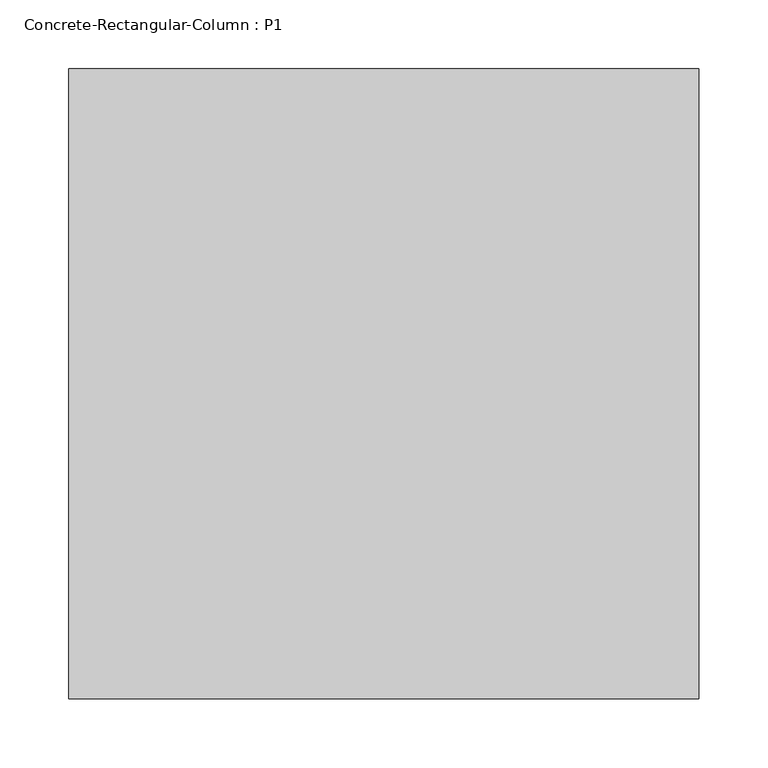
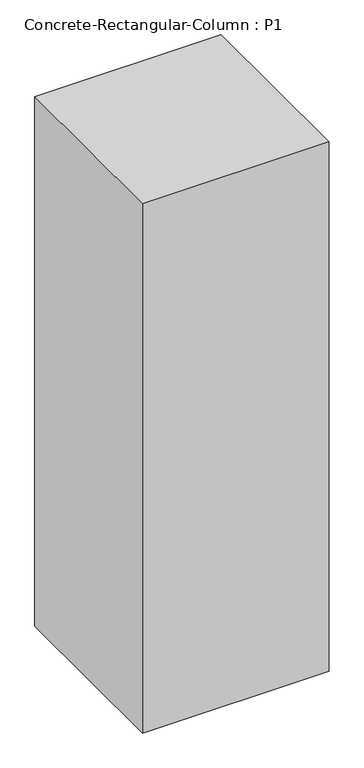
"""IFC4 building model written with IfcOpenShell, lengths in millimetres: column geometry, Concrete-Rectangular-Column : P1."""

from ifc_helpers import new_model, si_unit, frame, origin, place, context, project, spatial, polyline, outline, extrude, source, transform, mapped, element, save


def concrete_rectangular_column_p1_c4786f08(model_context):
    return source(origin(), model_context, "Body", "SweptSolid", [
        extrude(outline(polyline([(228.6, 228.6), (228.6, -228.6), (-228.6, -228.6), (-228.6, 228.6), (228.6, 228.6)])), frame((0.0, 0.0, -1371.6), z_axis=(0.0, 0.0, 1.0), x_axis=(1.0, 0.0, 0.0)), (0.0, 0.0, 1.0), 1371.6),
    ])


if __name__ == "__main__":
    model = new_model("IFC4")
    model_context = context("Model", 3, world=origin())
    ifc_project = project(units=[si_unit("LENGTHUNIT", "METRE", prefix="MILLI")], contexts=[model_context])
    site = spatial("IfcSite", under=ifc_project)
    building = spatial("IfcBuilding", under=site)
    placement = place(None, origin())
    concrete_rectangular_column_p1_shape = concrete_rectangular_column_p1_c4786f08(model_context)
    element("IfcColumn", 1, ObjectType="Concrete-Rectangular-Column : P1", at=placement, inside=building, context=model_context, shape_type="MappedRepresentation", body=[
        mapped(concrete_rectangular_column_p1_shape, transform((0.0, 0.0, 0.0), x_axis=(1.0, 0.0, 0.0), y_axis=(0.0, 1.0, 0.0), z_axis=(0.0, 0.0, 1.0))),
    ])
    save(model, "model.ifc")

# Revit data of these elements
# Type "Concrete-Rectangular-Column : P1"
#   Assembly Code = "B10"
#   b = 1' - 6"
#   h = 1' - 6"
#   Structural Material [instance default] = Concrete, Cast-in-Place gray
# Element 1 (IfcColumn, "Concrete-Rectangular-Column : P1")
#   Materials on its faces: "Concrete, Cast-in-Place gray"
# Materials
#   "Concrete, Cast-in-Place gray": class "Concrete", colour RGB 192 192 192, transparency 0, Description = "Cast-in-place concrete", Cost = 0
